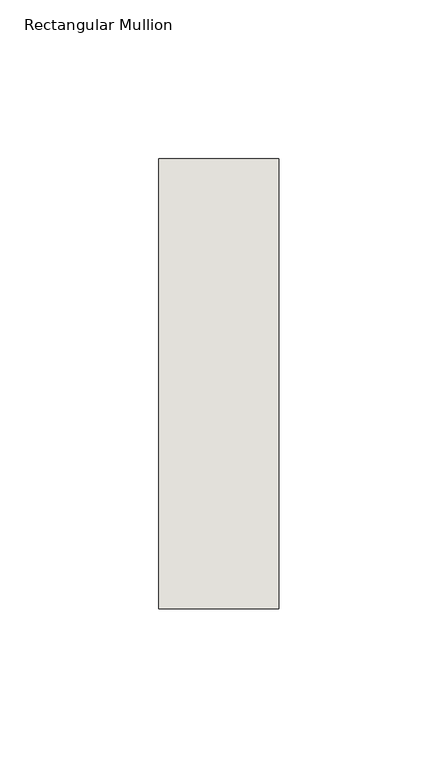
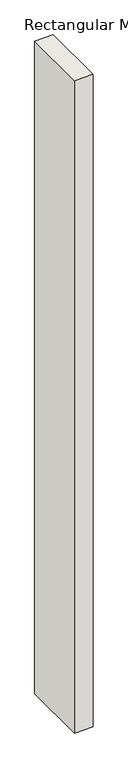
"""IFC4 building model written with IfcOpenShell, lengths in millimetres: wall geometry, Rectangular Mullion : NLRS_21_CWM_hsb-regel 38x142_gen_rsf."""

from ifc_helpers import new_model, si_unit, frame, origin, place, context, project, spatial, polyline, outline, extrude, source, transform, mapped, element, save


def rectangular_mullion_d24150c1(model_context):
    return source(origin(), model_context, "Body", "SweptSolid", [
        extrude(outline(polyline([(19.0, -71.0), (-19.0, -71.0), (-19.0, 71.0), (19.0, 71.0), (19.0, -71.0)])), frame((0.0, 0.0, -1421.0), z_axis=(0.0, 0.0, 1.0), x_axis=(1.0, 0.0, 0.0)), (0.0, 0.0, 1.0), 1421.0),
    ])


if __name__ == "__main__":
    model = new_model("IFC4")
    model_context = context("Model", 3, world=origin())
    ifc_project = project(units=[si_unit("LENGTHUNIT", "METRE", prefix="MILLI")], contexts=[model_context])
    site = spatial("IfcSite", under=ifc_project)
    building = spatial("IfcBuilding", under=site)
    placement = place(None, origin())
    rectangular_mullion_shape = rectangular_mullion_d24150c1(model_context)
    element("IfcWall", 1, ObjectType="Rectangular Mullion : NLRS_21_CWM_hsb-regel 38x142_gen_rsf", at=placement, inside=building, context=model_context, shape_type="MappedRepresentation", body=[
        mapped(rectangular_mullion_shape, transform((0.0, 0.0, 0.0), x_axis=(1.0, 0.0, 0.0), y_axis=(0.0, 1.0, 0.0), z_axis=(0.0, 0.0, 1.0))),
    ])
    save(model, "model.ifc")

# Revit data of these elements
# Type "Rectangular Mullion : NLRS_21_CWM_hsb-regel 38x142_gen_rsf"
#   Type IfcGUID = "07M7mRoiH1CR8m_RSKIwpF"
#   Assembly Code = "21.10"
#   IfcExportAs = "IfcWall"
#   built-in parameter 1007322 = 0.465879 (stored number, unit not read)
#   built-in parameter 1007321 = 0.062336 (stored number, unit not read)
#   built-in parameter 1007320 = 0.062336 (stored number, unit not read)
# Element 1 (IfcWall, "Rectangular Mullion : NLRS_21_CWM_hsb-regel 38x142_gen_rsf")
#   Materials on its faces: "NLRS_i2_hout naaldhout vuren_gen_rsf"
# Materials
#   "NLRS_i2_hout naaldhout vuren_gen_rsf": class "I - Hout", colour RGB 234 199 147, transparency 0, Keynote = "i2", Manufacturer = "Revit Standards Foundation", URL = "www.revitstandards.org", Description = "hout vuren", Cost = 0
